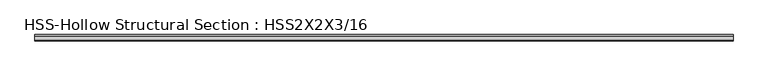
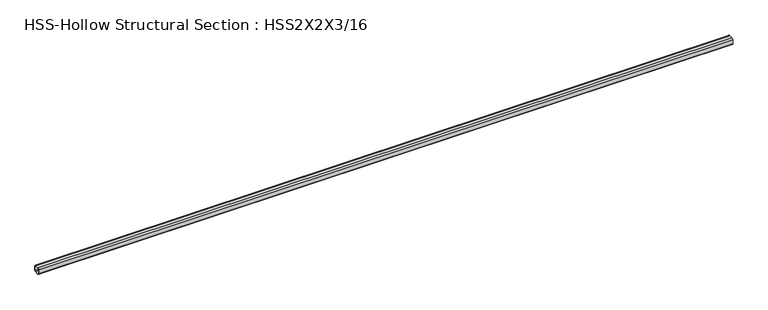
"""IFC4 building model written with IfcOpenShell, lengths in millimetres: beam geometry, HSS-Hollow Structural Section : HSS2X2X3/16."""

import ifcopenshell
import ifcopenshell.guid

model = None  # the IFC model being written
_history = None  # IfcOwnerHistory: only IFC2X3 demands one
_inside = {}  # id of a spatial element -> (the spatial element, [elements in it])
_under = {}  # id of a project, library or spatial element -> (it, [spatial elements below it])
_declared = {}  # id of a project -> (the project, [libraries it declares])
_typed = {}  # id of a type object -> (the type object, [elements of that type])
_made_of = {}  # id of a material, layer set ... -> (it, [elements and type objects made of it])


def new_model(schema):
    """Start an empty IFC model of exactly this schema.

    Asked for "IFC4X3", IfcOpenShell would pick the latest addendum, in which some entities
    have other attributes; the version numbers below select the first issue.
    IFC2X3 requires an IfcOwnerHistory on every rooted entity: one is made here for all.
    """
    global model, _history
    if schema == "IFC4X3":
        model = ifcopenshell.file(schema_version=(4, 3, 0, 0))
    else:
        model = ifcopenshell.file(schema=schema)
    _inside.clear()
    _under.clear()
    _declared.clear()
    _typed.clear()
    _made_of.clear()
    _history = None
    if model.schema == "IFC2X3":
        org = make("IfcOrganization", Name="unknown")
        user = make(
            "IfcPersonAndOrganization",
            ThePerson=make("IfcPerson", FamilyName="unknown"),
            TheOrganization=org,
        )
        app = make(
            "IfcApplication",
            ApplicationDeveloper=org,
            Version="unknown",
            ApplicationFullName="unknown",
            ApplicationIdentifier="unknown",
        )
        _history = make(
            "IfcOwnerHistory",
            OwningUser=user,
            OwningApplication=app,
            ChangeAction="ADDED",
            CreationDate=0,
        )
    return model


def make(cls, **values):
    """One entity of the class cls with the attributes given. An attribute that is None is left unset."""
    return model.create_entity(
        cls, **{name: value for name, value in values.items() if value is not None}
    )


def rooted(cls, **values):
    """An entity with a GlobalId (a new one), such as an element, a storey or a relation."""
    return make(cls, GlobalId=ifcopenshell.guid.new(), OwnerHistory=_history, **values)


def si_unit(unit_type, name, prefix=None):
    """IfcSIUnit, for example si_unit("LENGTHUNIT", "METRE", prefix="MILLI")."""
    return make("IfcSIUnit", UnitType=unit_type, Prefix=prefix, Name=name)


def assignment(units):
    """IfcUnitAssignment: the units of a project."""
    return None if units is None else make("IfcUnitAssignment", Units=units)


def point(xyz):
    """IfcCartesianPoint."""
    return None if xyz is None else make("IfcCartesianPoint", Coordinates=xyz)


def direction(xyz):
    """IfcDirection."""
    return None if xyz is None else make("IfcDirection", DirectionRatios=xyz)


def frame(location, z_axis=None, x_axis=None):
    """IfcAxis2Placement3D, a coordinate frame: its origin and axes. An axis left out is left unset."""
    return make(
        "IfcAxis2Placement3D",
        Location=point(location),
        Axis=direction(z_axis),
        RefDirection=direction(x_axis),
    )


def frame_2d(location, x_axis=None):
    """IfcAxis2Placement2D, a coordinate frame in the plane: its origin and x axis."""
    return make(
        "IfcAxis2Placement2D", Location=point(location), RefDirection=direction(x_axis)
    )


def origin():
    """The frame at (0, 0, 0) with its axes left unset."""
    return frame((0.0, 0.0, 0.0))


def place(relative_to, where):
    """IfcLocalPlacement: puts the frame where relative to a parent placement (None: the world)."""
    return make(
        "IfcLocalPlacement", PlacementRelTo=relative_to, RelativePlacement=where
    )


def context(
    kind, dimensions, precision=None, world=None, true_north=None, identifier=None
):
    """IfcGeometricRepresentationContext, for example the 3D "Model" context."""
    return make(
        "IfcGeometricRepresentationContext",
        ContextIdentifier=identifier,
        ContextType=kind,
        CoordinateSpaceDimension=dimensions,
        Precision=precision,
        WorldCoordinateSystem=world,
        TrueNorth=true_north,
    )


def project(units=None, contexts=None):
    """IfcProject with its units and contexts."""
    return rooted(
        "IfcProject",
        Name="project",
        RepresentationContexts=contexts,
        UnitsInContext=assignment(units),
    )


def spatial(cls, under=None, at=None, **own):
    """A site, building, storey or space (cls), placed at a placement, below another one or the project."""
    s = rooted(cls, ObjectPlacement=at, **own)
    if under is not None:
        _under.setdefault(under.id(), (under, []))[1].append(s)
    return s


def polyline(points):
    """IfcPolyline through the points."""
    return make("IfcPolyline", Points=[point(p) for p in points])


def circle_curve(where, radius):
    """IfcCircle in the frame where."""
    return make("IfcCircle", Position=where, Radius=radius)


def trimmed(basis, trim1, trim2, sense, master):
    """IfcTrimmedCurve: the piece of a basis curve between two trims."""
    return make(
        "IfcTrimmedCurve",
        BasisCurve=basis,
        Trim1=trim1,
        Trim2=trim2,
        SenseAgreement=sense,
        MasterRepresentation=master,
    )


def segment(curve, same_sense, transition):
    """IfcCompositeCurveSegment."""
    return make(
        "IfcCompositeCurveSegment",
        Transition=transition,
        SameSense=same_sense,
        ParentCurve=curve,
    )


def composite_curve(segments, self_intersect=None):
    """IfcCompositeCurve: segments joined end to end."""
    return make("IfcCompositeCurve", Segments=segments, SelfIntersect=self_intersect)


def outline(outer, holes=None, kind="AREA"):
    """IfcArbitraryClosedProfileDef: a profile drawn as a closed curve; with holes, ...WithVoids."""
    if holes is None:
        return make("IfcArbitraryClosedProfileDef", ProfileType=kind, OuterCurve=outer)
    return make(
        "IfcArbitraryProfileDefWithVoids",
        ProfileType=kind,
        OuterCurve=outer,
        InnerCurves=holes,
    )


def extrude(swept, where, along, depth):
    """IfcExtrudedAreaSolid: the profile swept, set in the frame where, extruded along a direction by depth."""
    return make(
        "IfcExtrudedAreaSolid",
        SweptArea=swept,
        Position=where,
        ExtrudedDirection=direction(along),
        Depth=depth,
    )


def shape(context_of_items, identifier, shape_type, items):
    """IfcShapeRepresentation: the items that make up one representation, for example the "Body"."""
    return make(
        "IfcShapeRepresentation",
        ContextOfItems=context_of_items,
        RepresentationIdentifier=identifier,
        RepresentationType=shape_type,
        Items=items,
    )


def source(mapping_origin, context_of_items, identifier, shape_type, items):
    """IfcRepresentationMap: a shape defined once, which mapped items show again and again."""
    return make(
        "IfcRepresentationMap",
        MappingOrigin=mapping_origin,
        MappedRepresentation=shape(context_of_items, identifier, shape_type, items),
    )


def transform(
    local_origin,
    x_axis=None,
    y_axis=None,
    z_axis=None,
    scale=None,
    scale2=None,
    scale3=None,
    uniform=True,
):
    """IfcCartesianTransformationOperator3D, or its non-uniform kind. x_axis, y_axis, z_axis: its Axis1, 2, 3."""
    if uniform:
        return make(
            "IfcCartesianTransformationOperator3D",
            Axis1=direction(x_axis),
            Axis2=direction(y_axis),
            LocalOrigin=point(local_origin),
            Scale=scale,
            Axis3=direction(z_axis),
        )
    return make(
        "IfcCartesianTransformationOperator3DnonUniform",
        Axis1=direction(x_axis),
        Axis2=direction(y_axis),
        LocalOrigin=point(local_origin),
        Scale=scale,
        Axis3=direction(z_axis),
        Scale2=scale2,
        Scale3=scale3,
    )


def mapped(mapping_source, mapping_target):
    """IfcMappedItem: shows the shape of a source again, moved by a transform."""
    return make(
        "IfcMappedItem", MappingSource=mapping_source, MappingTarget=mapping_target
    )


def made_of(thing, what):
    """Note that an element or type object is made of a material, layer set ...; save() writes the relation."""
    if what is not None:
        _made_of.setdefault(what.id(), (what, []))[1].append(thing)
    return thing


def element(
    cls,
    number,
    at=None,
    inside=None,
    cuts=None,
    type_object=None,
    material=None,
    context=None,
    identifier="Body",
    shape_type=None,
    held_by="IfcProductDefinitionShape",
    body=None,
    shapes=None,
    **own,
):
    """One element of the class cls, such as IfcWall. Its Tag is "e" and its number.

    at: its placement. inside: the storey or other place that contains it. cuts: it is an
    opening in that element (IfcRelVoidsElement). A single representation is given by context,
    identifier, shape_type and body (its items); several are given by shapes. held_by: the class
    of the entity that holds the representations. save() writes the other relations.
    """
    e = rooted(cls, Tag="e%d" % number, ObjectPlacement=at, **own)
    if body is not None:
        shapes = [shape(context, identifier, shape_type, body)]
    if shapes is not None:
        e.Representation = make(held_by, Representations=shapes)
    if inside is not None:
        _inside.setdefault(inside.id(), (inside, []))[1].append(e)
    if cuts is not None:
        rooted(
            "IfcRelVoidsElement", RelatingBuildingElement=cuts, RelatedOpeningElement=e
        )
    if type_object is not None:
        _typed.setdefault(type_object.id(), (type_object, []))[1].append(e)
    return made_of(e, material)


def aggregate(whole, parts):
    """IfcRelAggregates: a whole, such as a stair, and the parts it consists of."""
    return rooted("IfcRelAggregates", RelatingObject=whole, RelatedObjects=parts)


def save(model, path):
    """Write the relations noted so far, then the file.

    IfcRelAggregates (storeys below a building ...), IfcRelContainedInSpatialStructure (elements
    in a storey), IfcRelDefinesByType, IfcRelAssociatesMaterial and IfcRelDeclares: one each for
    every whole, place, type object, material and project.
    """
    for whole, parts in _under.values():
        aggregate(whole, parts)
    for where, things in _inside.values():
        rooted(
            "IfcRelContainedInSpatialStructure",
            RelatedElements=things,
            RelatingStructure=where,
        )
    for kind, things in _typed.values():
        rooted("IfcRelDefinesByType", RelatedObjects=things, RelatingType=kind)
    for what, things in _made_of.values():
        rooted("IfcRelAssociatesMaterial", RelatedObjects=things, RelatingMaterial=what)
    for by, libraries in _declared.values():
        rooted("IfcRelDeclares", RelatingContext=by, RelatedDefinitions=libraries)
    model.write(path)


def hss_hollow_structural_section_hss2x2x3_16_21cd95f6(model_context):
    return source(origin(), model_context, "Body", "SweptSolid", [
        extrude(outline(composite_curve([segment(polyline([(25.4, 16.5608), (25.4, -16.5608)]), True, "CONTINUOUS"), segment(trimmed(circle_curve(frame_2d((16.5608, -16.5608)), 8.8392), [point((25.4, -16.5608))], [point((16.5608, -25.4))], False, "CARTESIAN"), True, "CONTINUOUS"), segment(polyline([(16.5608, -25.4), (-16.5608, -25.4)]), True, "CONTINUOUS"), segment(trimmed(circle_curve(frame_2d((-16.5608, -16.5608)), 8.8392), [point((-16.5608, -25.4))], [point((-25.4, -16.5608))], False, "CARTESIAN"), True, "CONTINUOUS"), segment(polyline([(-25.4, -16.5608), (-25.4, 16.5608)]), True, "CONTINUOUS"), segment(trimmed(circle_curve(frame_2d((-16.5608, 16.5608)), 8.8392), [point((-25.4, 16.5608))], [point((-16.5608, 25.4))], False, "CARTESIAN"), True, "CONTINUOUS"), segment(polyline([(-16.5608, 25.4), (16.5608, 25.4)]), True, "CONTINUOUS"), segment(trimmed(circle_curve(frame_2d((16.5608, 16.5608)), 8.8392), [point((16.5608, 25.4))], [point((25.4, 16.5608))], False, "CARTESIAN"), True, "CONTINUOUS")], self_intersect=False), holes=[composite_curve([segment(trimmed(circle_curve(frame_2d((-16.5608, 16.5608)), 4.4196), [point((-16.5608, 20.9804))], [point((-20.9804, 16.5608))], True, "CARTESIAN"), True, "CONTINUOUS"), segment(polyline([(-20.9804, 16.5608), (-20.9804, -16.5608)]), True, "CONTINUOUS"), segment(trimmed(circle_curve(frame_2d((-16.5608, -16.5608)), 4.4196), [point((-20.9804, -16.5608))], [point((-16.5608, -20.9804))], True, "CARTESIAN"), True, "CONTINUOUS"), segment(polyline([(-16.5608, -20.9804), (16.5608, -20.9804)]), True, "CONTINUOUS"), segment(trimmed(circle_curve(frame_2d((16.5608, -16.5608)), 4.4196), [point((16.5608, -20.9804))], [point((20.9804, -16.5608))], True, "CARTESIAN"), True, "CONTINUOUS"), segment(polyline([(20.9804, -16.5608), (20.9804, 16.5608)]), True, "CONTINUOUS"), segment(trimmed(circle_curve(frame_2d((16.5608, 16.5608)), 4.4196), [point((20.9804, 16.5608))], [point((16.5608, 20.9804))], True, "CARTESIAN"), True, "CONTINUOUS"), segment(polyline([(16.5608, 20.9804), (-16.5608, 20.9804)]), True, "CONTINUOUS")], self_intersect=False)]), frame((4003.675, 0.0, 0.0), z_axis=(1.0, 0.0, 0.0), x_axis=(0.0, 1.0, 0.0)), (0.0, 0.0, 1.0), 5458.61875),
    ])


if __name__ == "__main__":
    model = new_model("IFC4")
    model_context = context("Model", 3, world=origin())
    ifc_project = project(units=[si_unit("LENGTHUNIT", "METRE", prefix="MILLI")], contexts=[model_context])
    site = spatial("IfcSite", under=ifc_project)
    building = spatial("IfcBuilding", under=site)
    placement = place(None, origin())
    hss_hollow_structural_section_hss2x2x3_16_shape = hss_hollow_structural_section_hss2x2x3_16_21cd95f6(model_context)
    element("IfcBeam", 1, ObjectType="HSS-Hollow Structural Section : HSS2X2X3/16", at=placement, inside=building, context=model_context, shape_type="MappedRepresentation", body=[
        mapped(hss_hollow_structural_section_hss2x2x3_16_shape, transform((0.0, 0.0, 0.0), x_axis=(1.0, 0.0, 0.0), y_axis=(0.0, 1.0, 0.0), z_axis=(0.0, 0.0, 1.0))),
    ])
    save(model, "model.ifc")

# Revit data of these elements
# Type "HSS-Hollow Structural Section : HSS2X2X3/16"
#   Keynote = "M05121300.04"
#   Assembly Code = "B10"
#   Shape = "Square"
#   W = 4.3
#   Ht = 0' - 2"
#   Length [instance default] = 5' - 0"
#   b = 0' - 2"
#   kr = 0' - 0.348"
#   t = 0' - 0.174"
#   A = 0.00826389 SF
#   Structural Material [instance default] = Steel ASTM A500, Grade B, Rectangular and Square
# Element 1 (IfcBeam, "HSS-Hollow Structural Section : HSS2X2X3/16")
#   Materials on its faces: "Steel ASTM A500, Grade B, Rectangular and Square"
# Materials
#   "Steel ASTM A500, Grade B, Rectangular and Square": class "Metal", colour RGB 199 199 199, transparency 0, Description = "Carbon steel", Cost = 0
